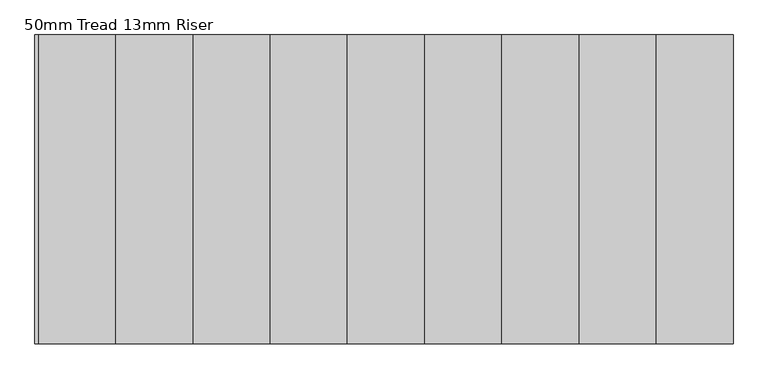
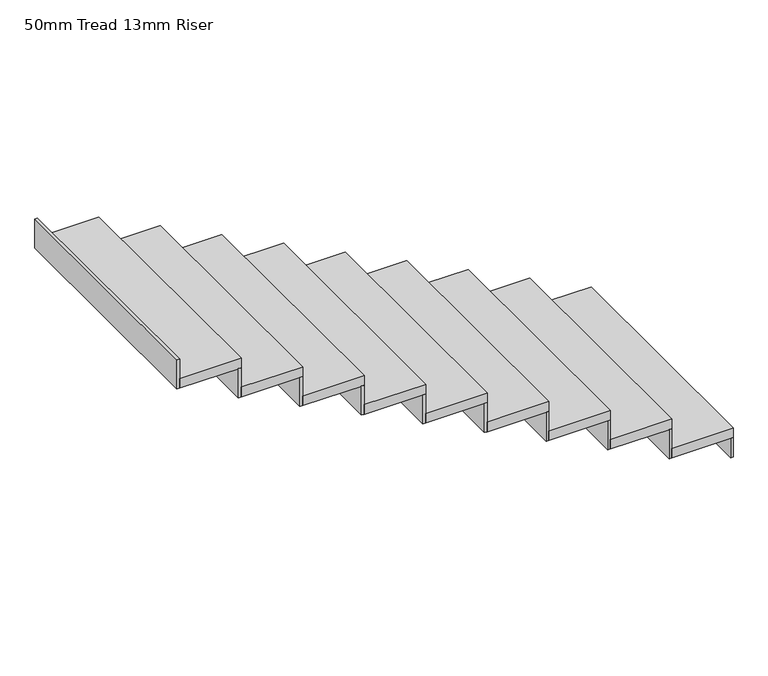
"""IFC4 building model written with IfcOpenShell, lengths in millimetres: stair flight geometry, 50mm Tread 13mm Riser."""

from ifc_helpers import new_model, si_unit, frame, origin, origin_with_axes, place, context, project, spatial, polyline, outline, extrude, source, transform, mapped, element, save


def stair_flight_50mm_tread_13mm_riser_f0f57eae(model_context):
    return source(origin(), model_context, "Body", "SweptSolid", [
        extrude(outline(polyline([(22437.0372571, -4900.9614996), (22449.5372571, -4900.9614996), (22449.5372571, -6100.9614996), (22437.0372571, -6100.9614996), (22437.0372571, -4900.9614996)])), origin_with_axes(), (0.0, 0.0, 1.0), 100.0),
        extrude(outline(polyline([(22149.5372571, -6100.9614996), (22149.5372571, -4900.9614996), (22449.5372571, -4900.9614996), (22449.5372571, -6100.9614996), (22149.5372571, -6100.9614996)])), frame((0.0, 0.0, 100.0), z_axis=(0.0, 0.0, 1.0), x_axis=(1.0, 0.0, 0.0)), (0.0, 0.0, 1.0), 50.0),
        extrude(outline(polyline([(22137.0372571, -4900.9614996), (22149.5372571, -4900.9614996), (22149.5372571, -6100.9614996), (22137.0372571, -6100.9614996), (22137.0372571, -4900.9614996)])), frame((0.0, 0.0, 100.0), z_axis=(0.0, 0.0, 1.0), x_axis=(1.0, 0.0, 0.0)), (0.0, 0.0, 1.0), 150.0),
        extrude(outline(polyline([(21849.5372571, -6100.9614996), (21849.5372571, -4900.9614996), (22149.5372571, -4900.9614996), (22149.5372571, -6100.9614996), (21849.5372571, -6100.9614996)])), frame((0.0, 0.0, 250.0), z_axis=(0.0, 0.0, 1.0), x_axis=(1.0, 0.0, 0.0)), (0.0, 0.0, 1.0), 50.0),
        extrude(outline(polyline([(21837.0372571, -4900.9614996), (21849.5372571, -4900.9614996), (21849.5372571, -6100.9614996), (21837.0372571, -6100.9614996), (21837.0372571, -4900.9614996)])), frame((0.0, 0.0, 250.0), z_axis=(0.0, 0.0, 1.0), x_axis=(1.0, 0.0, 0.0)), (0.0, 0.0, 1.0), 150.0),
        extrude(outline(polyline([(21549.5372571, -6100.9614996), (21549.5372571, -4900.9614996), (21849.5372571, -4900.9614996), (21849.5372571, -6100.9614996), (21549.5372571, -6100.9614996)])), frame((0.0, 0.0, 400.0), z_axis=(0.0, 0.0, 1.0), x_axis=(1.0, 0.0, 0.0)), (0.0, 0.0, 1.0), 50.0),
        extrude(outline(polyline([(21537.0372571, -4900.9614996), (21549.5372571, -4900.9614996), (21549.5372571, -6100.9614996), (21537.0372571, -6100.9614996), (21537.0372571, -4900.9614996)])), frame((0.0, 0.0, 400.0), z_axis=(0.0, 0.0, 1.0), x_axis=(1.0, 0.0, 0.0)), (0.0, 0.0, 1.0), 150.0),
        extrude(outline(polyline([(21249.5372571, -6100.9614996), (21249.5372571, -4900.9614996), (21549.5372571, -4900.9614996), (21549.5372571, -6100.9614996), (21249.5372571, -6100.9614996)])), frame((0.0, 0.0, 550.0), z_axis=(0.0, 0.0, 1.0), x_axis=(1.0, 0.0, 0.0)), (0.0, 0.0, 1.0), 50.0),
        extrude(outline(polyline([(21237.0372571, -4900.9614996), (21249.5372571, -4900.9614996), (21249.5372571, -6100.9614996), (21237.0372571, -6100.9614996), (21237.0372571, -4900.9614996)])), frame((0.0, 0.0, 550.0), z_axis=(0.0, 0.0, 1.0), x_axis=(1.0, 0.0, 0.0)), (0.0, 0.0, 1.0), 150.0),
        extrude(outline(polyline([(20949.5372571, -6100.9614996), (20949.5372571, -4900.9614996), (21249.5372571, -4900.9614996), (21249.5372571, -6100.9614996), (20949.5372571, -6100.9614996)])), frame((0.0, 0.0, 700.0), z_axis=(0.0, 0.0, 1.0), x_axis=(1.0, 0.0, 0.0)), (0.0, 0.0, 1.0), 50.0),
        extrude(outline(polyline([(20937.0372571, -4900.9614996), (20949.5372571, -4900.9614996), (20949.5372571, -6100.9614996), (20937.0372571, -6100.9614996), (20937.0372571, -4900.9614996)])), frame((0.0, 0.0, 700.0), z_axis=(0.0, 0.0, 1.0), x_axis=(1.0, 0.0, 0.0)), (0.0, 0.0, 1.0), 150.0),
        extrude(outline(polyline([(20649.5372571, -6100.9614996), (20649.5372571, -4900.9614996), (20949.5372571, -4900.9614996), (20949.5372571, -6100.9614996), (20649.5372571, -6100.9614996)])), frame((0.0, 0.0, 850.0), z_axis=(0.0, 0.0, 1.0), x_axis=(1.0, 0.0, 0.0)), (0.0, 0.0, 1.0), 50.0),
        extrude(outline(polyline([(20637.0372571, -4900.9614996), (20649.5372571, -4900.9614996), (20649.5372571, -6100.9614996), (20637.0372571, -6100.9614996), (20637.0372571, -4900.9614996)])), frame((0.0, 0.0, 850.0), z_axis=(0.0, 0.0, 1.0), x_axis=(1.0, 0.0, 0.0)), (0.0, 0.0, 1.0), 150.0),
        extrude(outline(polyline([(20349.5372571, -6100.9614996), (20349.5372571, -4900.9614996), (20649.5372571, -4900.9614996), (20649.5372571, -6100.9614996), (20349.5372571, -6100.9614996)])), frame((0.0, 0.0, 1000.0), z_axis=(0.0, 0.0, 1.0), x_axis=(1.0, 0.0, 0.0)), (0.0, 0.0, 1.0), 50.0),
        extrude(outline(polyline([(20337.0372571, -4900.9614996), (20349.5372571, -4900.9614996), (20349.5372571, -6100.9614996), (20337.0372571, -6100.9614996), (20337.0372571, -4900.9614996)])), frame((0.0, 0.0, 1000.0), z_axis=(0.0, 0.0, 1.0), x_axis=(1.0, 0.0, 0.0)), (0.0, 0.0, 1.0), 150.0),
        extrude(outline(polyline([(20049.5372571, -6100.9614996), (20049.5372571, -4900.9614996), (20349.5372571, -4900.9614996), (20349.5372571, -6100.9614996), (20049.5372571, -6100.9614996)])), frame((0.0, 0.0, 1150.0), z_axis=(0.0, 0.0, 1.0), x_axis=(1.0, 0.0, 0.0)), (0.0, 0.0, 1.0), 50.0),
        extrude(outline(polyline([(20037.0372571, -4900.9614996), (20049.5372571, -4900.9614996), (20049.5372571, -6100.9614996), (20037.0372571, -6100.9614996), (20037.0372571, -4900.9614996)])), frame((0.0, 0.0, 1150.0), z_axis=(0.0, 0.0, 1.0), x_axis=(1.0, 0.0, 0.0)), (0.0, 0.0, 1.0), 150.0),
        extrude(outline(polyline([(19737.0372571, -4900.9614996), (19749.5372571, -4900.9614996), (19749.5372571, -6100.9614996), (19737.0372571, -6100.9614996), (19737.0372571, -4900.9614996)])), frame((0.0, 0.0, 1300.0), z_axis=(0.0, 0.0, 1.0), x_axis=(1.0, 0.0, 0.0)), (0.0, 0.0, 1.0), 150.0),
        extrude(outline(polyline([(19749.5372571, -6100.9614996), (19749.5372571, -4900.9614996), (20049.5372571, -4900.9614996), (20049.5372571, -6100.9614996), (19749.5372571, -6100.9614996)])), frame((0.0, 0.0, 1300.0), z_axis=(0.0, 0.0, 1.0), x_axis=(1.0, 0.0, 0.0)), (0.0, 0.0, 1.0), 50.0),
    ])


if __name__ == "__main__":
    model = new_model("IFC4")
    model_context = context("Model", 3, world=origin())
    ifc_project = project(units=[si_unit("LENGTHUNIT", "METRE", prefix="MILLI")], contexts=[model_context])
    site = spatial("IfcSite", under=ifc_project)
    building = spatial("IfcBuilding", under=site)
    placement = place(None, origin())
    stair_flight_50mm_tread_13mm_riser_shape = stair_flight_50mm_tread_13mm_riser_f0f57eae(model_context)
    element("IfcStairFlight", 1, ObjectType="50mm Tread 13mm Riser", at=placement, inside=building, context=model_context, shape_type="MappedRepresentation", body=[
        mapped(stair_flight_50mm_tread_13mm_riser_shape, transform((0.0, 0.0, 0.0), x_axis=(1.0, 0.0, 0.0), y_axis=(0.0, 1.0, 0.0), z_axis=(0.0, 0.0, 1.0))),
    ])
    save(model, "model.ifc")
